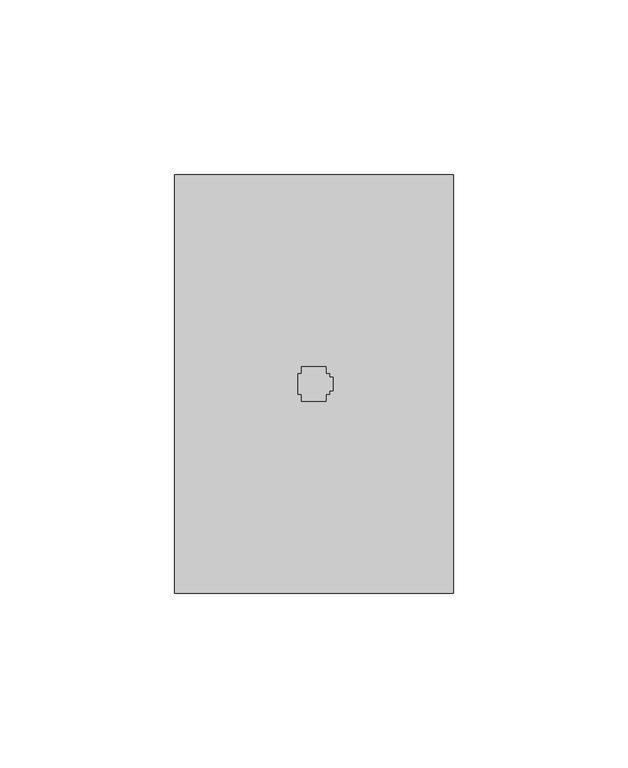
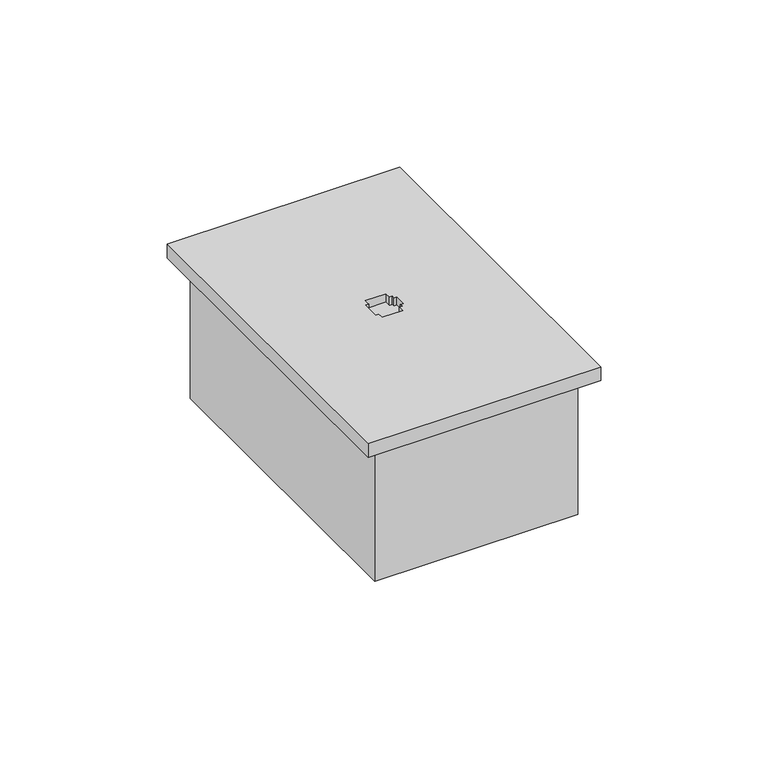
"""IFC4 building model written with IfcOpenShell, lengths in millimetres: proxy geometry, CAIXA VERTICE V7 : Telefone."""

from ifc_helpers import new_model, si_unit, origin, place, context, project, spatial, faceted_brep, source, transform, mapped, element, save


def electrical_fixtures_fc6e5b9e(model_context):
    return source(origin(), model_context, "Body", "Brep", [
        faceted_brep([(33.0, 1047.0, -48.0), (33.0, 1153.0, -48.0), (-33.0, 1153.0, -48.0), (-33.0, 1047.0, -48.0), (35.0, 1155.0, -50.0), (35.0, 1045.0, -50.0), (-35.0, 1045.0, -50.0), (-35.0, 1155.0, -50.0), (-35.0, 1155.0, 0.0), (35.0, 1155.0, 0.0), (-35.0, 1045.0, 0.0), (35.0, 1045.0, 0.0), (33.0, 1153.0, 0.0), (33.0, 1047.0, 0.0), (-33.0, 1047.0, 0.0), (-33.0, 1153.0, 0.0)], [[[0, 1, 2, 3]], [[4, 5, 6, 7]], [[4, 7, 8, 9]], [[8, 7, 6, 10]], [[10, 6, 5, 11]], [[11, 5, 4, 9]], [[9, 8, 10, 11], [12, 13, 14, 15]], [[13, 12, 1, 0]], [[14, 13, 0, 3]], [[15, 14, 3, 2]], [[12, 15, 2, 1]]]),
        faceted_brep([(40.0, 1160.0, 5.0), (-40.0, 1160.0, 5.0), (-40.0, 1040.0, 5.0), (40.0, 1040.0, 5.0), (-3.5, 1103.0, 5.0), (-3.5, 1105.0, 5.0), (3.5, 1105.0, 5.0), (3.5, 1103.0, 5.0), (4.5, 1103.0, 5.0), (4.5, 1102.0, 5.0), (5.5, 1102.0, 5.0), (5.5, 1098.0, 5.0), (4.5, 1098.0, 5.0), (4.5, 1097.0, 5.0), (3.5, 1097.0, 5.0), (3.5, 1095.0, 5.0), (-3.5, 1095.0, 5.0), (-3.5, 1097.0, 5.0), (-4.5, 1097.0, 5.0), (-4.5, 1103.0, 5.0), (-40.0, 1160.0, 0.0), (40.0, 1160.0, 0.0), (40.0, 1040.0, 0.0), (-40.0, 1040.0, 0.0), (-3.5, 1103.0, 2.0), (-3.5, 1105.0, 2.0), (-4.5, 1103.0, 2.0), (-4.5, 1097.0, 2.0), (-3.5, 1097.0, 2.0), (-3.5, 1095.0, 2.0), (3.5, 1095.0, 2.0), (3.5, 1097.0, 2.0), (3.5, 1105.0, 2.0), (4.5, 1097.0, 2.0), (4.5, 1098.0, 2.0), (5.5, 1098.0, 2.0), (5.5, 1102.0, 2.0), (4.5, 1102.0, 2.0), (4.5, 1103.0, 2.0), (3.5, 1103.0, 2.0)], [[[0, 1, 2, 3], [4, 5, 6, 7, 8, 9, 10, 11, 12, 13, 14, 15, 16, 17, 18, 19]], [[20, 21, 22, 23]], [[1, 0, 21, 20]], [[2, 1, 20, 23]], [[3, 2, 23, 22]], [[0, 3, 22, 21]], [[24, 25, 5, 4]], [[26, 24, 4, 19]], [[27, 26, 19, 18]], [[28, 27, 18, 17]], [[29, 28, 17, 16]], [[30, 29, 16, 15]], [[31, 30, 15, 14]], [[32, 25, 24, 26, 27, 28, 29, 30, 31, 33, 34, 35, 36, 37, 38, 39]], [[25, 32, 6, 5]], [[33, 31, 14, 13]], [[34, 33, 13, 12]], [[35, 34, 12, 11]], [[36, 35, 11, 10]], [[37, 36, 10, 9]], [[38, 37, 9, 8]], [[39, 38, 8, 7]], [[32, 39, 7, 6]]]),
    ])


if __name__ == "__main__":
    model = new_model("IFC4")
    model_context = context("Model", 3, world=origin())
    ifc_project = project(units=[si_unit("LENGTHUNIT", "METRE", prefix="MILLI")], contexts=[model_context])
    site = spatial("IfcSite", under=ifc_project)
    building = spatial("IfcBuilding", under=site)
    placement = place(None, origin())
    electrical_fixtures_shape = electrical_fixtures_fc6e5b9e(model_context)
    element("IfcBuildingElementProxy", 1, Name="CAIXA VERTICE V7 : Telefone", ObjectType="CAIXA VERTICE V7 : Telefone", at=placement, inside=building, context=model_context, shape_type="MappedRepresentation", body=[
        mapped(electrical_fixtures_shape, transform((0.0, 0.0, 0.0), x_axis=(1.0, 0.0, 0.0), y_axis=(0.0, 1.0, 0.0), z_axis=(0.0, 0.0, 1.0))),
    ])
    save(model, "model.ifc")

# Revit data of these elements
# Type "CAIXA VERTICE V7 : Telefone"
#   URL = "www.facebook.com/verticetreinamentos"
#   SEÇÃO [instance default] = ""
#   Rotação [instance default] = 0.00°
#   LARGURA DA TAMPA = 0.08 m
#   BORDA = 0.01 m
#   ALTURA DE INSTALAÇÃO [instance default] = 1.10 m
#   Distância Anotação [instance default] = 0.0015 m
#   ALTURA DA TAMPA = 0.12 m
#   Vertical [instance default] = yes
#   VER SEÇÃO [instance default] = no
#   SHADE ESQ [instance default] = no
#   SHADE DIR [instance default] = yes
#   HORIZONTAL [instance default] = no
#   ANDAR COM A LEGENDA [instance default] = 0
#   Material Tampa [instance default] = Plástico, branco opaco
#   Caixa = element 1798520
#   Anotação = element 1798519
#   Default Elevation = 0
# Element 1 (IfcBuildingElementProxy, "CAIXA VERTICE V7 : Telefone")
#   Materials on its faces: "Plástico, branco opaco"
# Materials
#   "Plástico, branco opaco": class "Plástico", colour RGB 120 120 120, transparency 0, Description = "Plastic, generic, opaque white", Cost = 0
